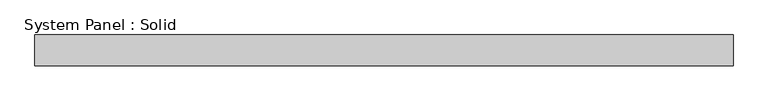
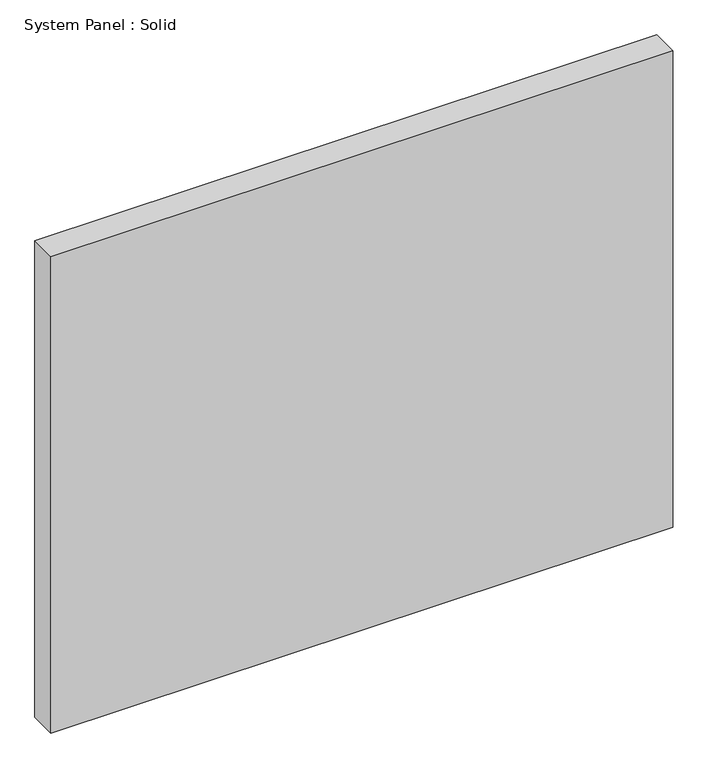
"""IFC4 building model written with IfcOpenShell, lengths in millimetres: plate geometry, System Panel : Solid."""

from ifc_helpers import new_model, si_unit, origin, origin_with_axes, place, context, project, spatial, polyline, outline, extrude, source, transform, mapped, element, save


def system_panel_solid_81e17396(model_context):
    return source(origin(), model_context, "Body", "SweptSolid", [
        extrude(outline(polyline([(713.3166666, -19.05), (-713.3166666, -19.05), (-713.3166666, 44.45), (713.3166666, 44.45), (713.3166666, -19.05)])), origin_with_axes(), (0.0, 0.0, 1.0), 1155.7),
    ])


if __name__ == "__main__":
    model = new_model("IFC4")
    model_context = context("Model", 3, world=origin())
    ifc_project = project(units=[si_unit("LENGTHUNIT", "METRE", prefix="MILLI")], contexts=[model_context])
    site = spatial("IfcSite", under=ifc_project)
    building = spatial("IfcBuilding", under=site)
    placement = place(None, origin())
    system_panel_solid_shape = system_panel_solid_81e17396(model_context)
    element("IfcPlate", 1, ObjectType="System Panel : Solid", at=placement, inside=building, context=model_context, shape_type="MappedRepresentation", body=[
        mapped(system_panel_solid_shape, transform((0.0, 0.0, 0.0), x_axis=(1.0, 0.0, 0.0), y_axis=(0.0, 1.0, 0.0), z_axis=(0.0, 0.0, 1.0))),
    ])
    save(model, "model.ifc")

# Revit data of these elements
# Type "System Panel : Solid"
#   Construction Type Id = "MDOOR"
#   Analytic Construction = "Metal"
#   Visual Light Transmittance = 0
#   Solar Heat Gain Coefficient = 0
#   Heat Transfer Coefficient (U) = 0.651978 BTU/(h·ft²·°F)
#   Define Thermal Properties by = 1
# Element 1 (IfcPlate, "System Panel : Solid")
#   Materials on its faces: "Default"
# Materials
#   "Default": class "Miscellaneous", colour RGB 127 127 127, transparency 0, Cost = 0
